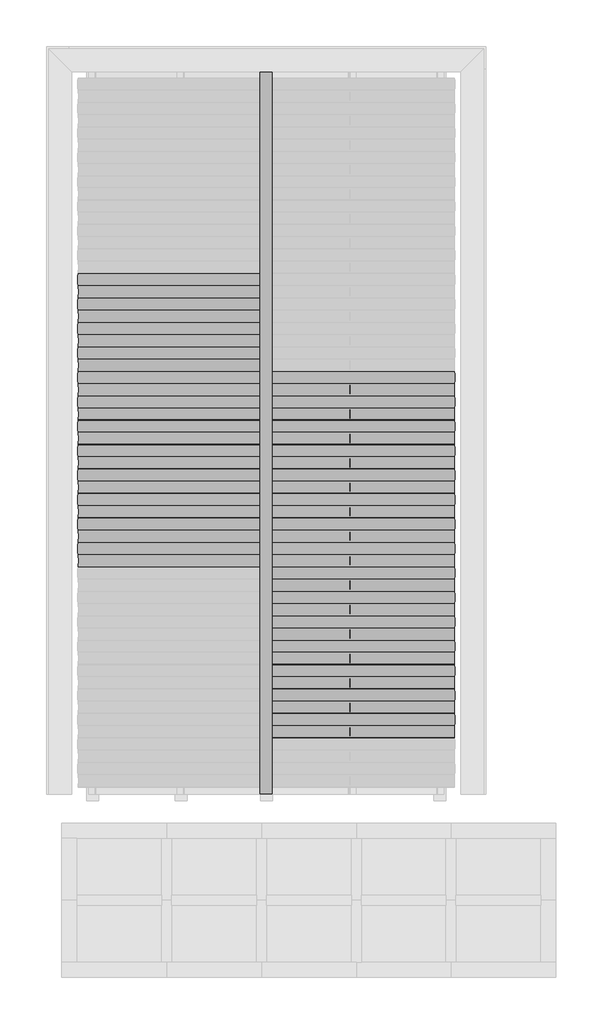
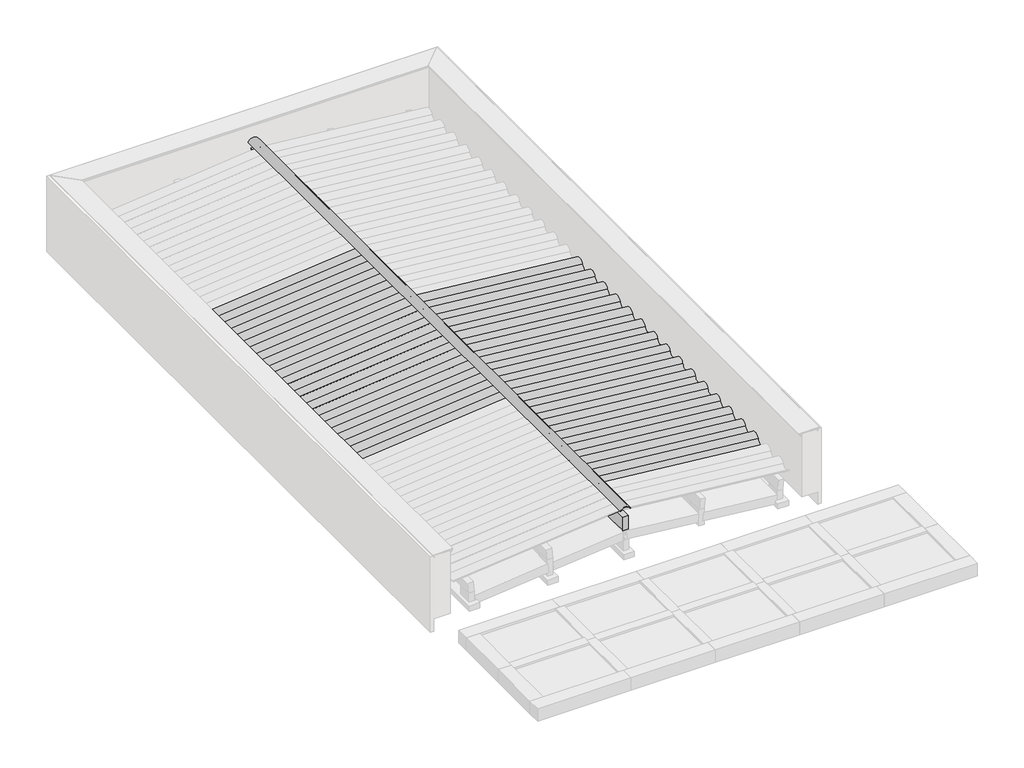
# One storey, part 2 of 3: 34 beams, 6 columns.
"""IFC4 building model written with IfcOpenShell, lengths in millimetres."""

import ifcopenshell
import ifcopenshell.guid

model = None  # the IFC model being written
_history = None  # IfcOwnerHistory: only IFC2X3 demands one
_inside = {}  # id of a spatial element -> (the spatial element, [elements in it])
_under = {}  # id of a project, library or spatial element -> (it, [spatial elements below it])
_declared = {}  # id of a project -> (the project, [libraries it declares])
_typed = {}  # id of a type object -> (the type object, [elements of that type])
_made_of = {}  # id of a material, layer set ... -> (it, [elements and type objects made of it])


def new_model(schema):
    """Start an empty IFC model of exactly this schema.

    Asked for "IFC4X3", IfcOpenShell would pick the latest addendum, in which some entities
    have other attributes; the version numbers below select the first issue.
    IFC2X3 requires an IfcOwnerHistory on every rooted entity: one is made here for all.
    """
    global model, _history
    if schema == "IFC4X3":
        model = ifcopenshell.file(schema_version=(4, 3, 0, 0))
    else:
        model = ifcopenshell.file(schema=schema)
    _inside.clear()
    _under.clear()
    _declared.clear()
    _typed.clear()
    _made_of.clear()
    _history = None
    if model.schema == "IFC2X3":
        org = make("IfcOrganization", Name="unknown")
        user = make(
            "IfcPersonAndOrganization",
            ThePerson=make("IfcPerson", FamilyName="unknown"),
            TheOrganization=org,
        )
        app = make(
            "IfcApplication",
            ApplicationDeveloper=org,
            Version="unknown",
            ApplicationFullName="unknown",
            ApplicationIdentifier="unknown",
        )
        _history = make(
            "IfcOwnerHistory",
            OwningUser=user,
            OwningApplication=app,
            ChangeAction="ADDED",
            CreationDate=0,
        )
    return model


def make(cls, **values):
    """One entity of the class cls with the attributes given. An attribute that is None is left unset."""
    return model.create_entity(
        cls, **{name: value for name, value in values.items() if value is not None}
    )


def rooted(cls, **values):
    """An entity with a GlobalId (a new one), such as an element, a storey or a relation."""
    return make(cls, GlobalId=ifcopenshell.guid.new(), OwnerHistory=_history, **values)


def si_unit(unit_type, name, prefix=None):
    """IfcSIUnit, for example si_unit("LENGTHUNIT", "METRE", prefix="MILLI")."""
    return make("IfcSIUnit", UnitType=unit_type, Prefix=prefix, Name=name)


def assignment(units):
    """IfcUnitAssignment: the units of a project."""
    return None if units is None else make("IfcUnitAssignment", Units=units)


def point(xyz):
    """IfcCartesianPoint."""
    return None if xyz is None else make("IfcCartesianPoint", Coordinates=xyz)


def direction(xyz):
    """IfcDirection."""
    return None if xyz is None else make("IfcDirection", DirectionRatios=xyz)


def frame(location, z_axis=None, x_axis=None):
    """IfcAxis2Placement3D, a coordinate frame: its origin and axes. An axis left out is left unset."""
    return make(
        "IfcAxis2Placement3D",
        Location=point(location),
        Axis=direction(z_axis),
        RefDirection=direction(x_axis),
    )


def frame_2d(location, x_axis=None):
    """IfcAxis2Placement2D, a coordinate frame in the plane: its origin and x axis."""
    return make(
        "IfcAxis2Placement2D", Location=point(location), RefDirection=direction(x_axis)
    )


def origin():
    """The frame at (0, 0, 0) with its axes left unset."""
    return frame((0.0, 0.0, 0.0))


def place(relative_to, where):
    """IfcLocalPlacement: puts the frame where relative to a parent placement (None: the world)."""
    return make(
        "IfcLocalPlacement", PlacementRelTo=relative_to, RelativePlacement=where
    )


def context(
    kind, dimensions, precision=None, world=None, true_north=None, identifier=None
):
    """IfcGeometricRepresentationContext, for example the 3D "Model" context."""
    return make(
        "IfcGeometricRepresentationContext",
        ContextIdentifier=identifier,
        ContextType=kind,
        CoordinateSpaceDimension=dimensions,
        Precision=precision,
        WorldCoordinateSystem=world,
        TrueNorth=true_north,
    )


def project(units=None, contexts=None):
    """IfcProject with its units and contexts."""
    return rooted(
        "IfcProject",
        Name="project",
        RepresentationContexts=contexts,
        UnitsInContext=assignment(units),
    )


def spatial(cls, under=None, at=None, **own):
    """A site, building, storey or space (cls), placed at a placement, below another one or the project."""
    s = rooted(cls, ObjectPlacement=at, **own)
    if under is not None:
        _under.setdefault(under.id(), (under, []))[1].append(s)
    return s


def polyline(points):
    """IfcPolyline through the points."""
    return make("IfcPolyline", Points=[point(p) for p in points])


def circle_curve(where, radius):
    """IfcCircle in the frame where."""
    return make("IfcCircle", Position=where, Radius=radius)


def trimmed(basis, trim1, trim2, sense, master):
    """IfcTrimmedCurve: the piece of a basis curve between two trims."""
    return make(
        "IfcTrimmedCurve",
        BasisCurve=basis,
        Trim1=trim1,
        Trim2=trim2,
        SenseAgreement=sense,
        MasterRepresentation=master,
    )


def segment(curve, same_sense, transition):
    """IfcCompositeCurveSegment."""
    return make(
        "IfcCompositeCurveSegment",
        Transition=transition,
        SameSense=same_sense,
        ParentCurve=curve,
    )


def composite_curve(segments, self_intersect=None):
    """IfcCompositeCurve: segments joined end to end."""
    return make("IfcCompositeCurve", Segments=segments, SelfIntersect=self_intersect)


def outline(outer, holes=None, kind="AREA"):
    """IfcArbitraryClosedProfileDef: a profile drawn as a closed curve; with holes, ...WithVoids."""
    if holes is None:
        return make("IfcArbitraryClosedProfileDef", ProfileType=kind, OuterCurve=outer)
    return make(
        "IfcArbitraryProfileDefWithVoids",
        ProfileType=kind,
        OuterCurve=outer,
        InnerCurves=holes,
    )


def extrude(swept, where, along, depth):
    """IfcExtrudedAreaSolid: the profile swept, set in the frame where, extruded along a direction by depth."""
    return make(
        "IfcExtrudedAreaSolid",
        SweptArea=swept,
        Position=where,
        ExtrudedDirection=direction(along),
        Depth=depth,
    )


def shape(context_of_items, identifier, shape_type, items):
    """IfcShapeRepresentation: the items that make up one representation, for example the "Body"."""
    return make(
        "IfcShapeRepresentation",
        ContextOfItems=context_of_items,
        RepresentationIdentifier=identifier,
        RepresentationType=shape_type,
        Items=items,
    )


def source(mapping_origin, context_of_items, identifier, shape_type, items):
    """IfcRepresentationMap: a shape defined once, which mapped items show again and again."""
    return make(
        "IfcRepresentationMap",
        MappingOrigin=mapping_origin,
        MappedRepresentation=shape(context_of_items, identifier, shape_type, items),
    )


def transform(
    local_origin,
    x_axis=None,
    y_axis=None,
    z_axis=None,
    scale=None,
    scale2=None,
    scale3=None,
    uniform=True,
):
    """IfcCartesianTransformationOperator3D, or its non-uniform kind. x_axis, y_axis, z_axis: its Axis1, 2, 3."""
    if uniform:
        return make(
            "IfcCartesianTransformationOperator3D",
            Axis1=direction(x_axis),
            Axis2=direction(y_axis),
            LocalOrigin=point(local_origin),
            Scale=scale,
            Axis3=direction(z_axis),
        )
    return make(
        "IfcCartesianTransformationOperator3DnonUniform",
        Axis1=direction(x_axis),
        Axis2=direction(y_axis),
        LocalOrigin=point(local_origin),
        Scale=scale,
        Axis3=direction(z_axis),
        Scale2=scale2,
        Scale3=scale3,
    )


def mapped(mapping_source, mapping_target):
    """IfcMappedItem: shows the shape of a source again, moved by a transform."""
    return make(
        "IfcMappedItem", MappingSource=mapping_source, MappingTarget=mapping_target
    )


def made_of(thing, what):
    """Note that an element or type object is made of a material, layer set ...; save() writes the relation."""
    if what is not None:
        _made_of.setdefault(what.id(), (what, []))[1].append(thing)
    return thing


def element(
    cls,
    number,
    at=None,
    inside=None,
    cuts=None,
    type_object=None,
    material=None,
    context=None,
    identifier="Body",
    shape_type=None,
    held_by="IfcProductDefinitionShape",
    body=None,
    shapes=None,
    **own,
):
    """One element of the class cls, such as IfcWall. Its Tag is "e" and its number.

    at: its placement. inside: the storey or other place that contains it. cuts: it is an
    opening in that element (IfcRelVoidsElement). A single representation is given by context,
    identifier, shape_type and body (its items); several are given by shapes. held_by: the class
    of the entity that holds the representations. save() writes the other relations.
    """
    e = rooted(cls, Tag="e%d" % number, ObjectPlacement=at, **own)
    if body is not None:
        shapes = [shape(context, identifier, shape_type, body)]
    if shapes is not None:
        e.Representation = make(held_by, Representations=shapes)
    if inside is not None:
        _inside.setdefault(inside.id(), (inside, []))[1].append(e)
    if cuts is not None:
        rooted(
            "IfcRelVoidsElement", RelatingBuildingElement=cuts, RelatedOpeningElement=e
        )
    if type_object is not None:
        _typed.setdefault(type_object.id(), (type_object, []))[1].append(e)
    return made_of(e, material)


def aggregate(whole, parts):
    """IfcRelAggregates: a whole, such as a stair, and the parts it consists of."""
    return rooted("IfcRelAggregates", RelatingObject=whole, RelatedObjects=parts)


def save(model, path):
    """Write the relations noted so far, then the file.

    IfcRelAggregates (storeys below a building ...), IfcRelContainedInSpatialStructure (elements
    in a storey), IfcRelDefinesByType, IfcRelAssociatesMaterial and IfcRelDeclares: one each for
    every whole, place, type object, material and project.
    """
    for whole, parts in _under.values():
        aggregate(whole, parts)
    for where, things in _inside.values():
        rooted(
            "IfcRelContainedInSpatialStructure",
            RelatedElements=things,
            RelatingStructure=where,
        )
    for kind, things in _typed.values():
        rooted("IfcRelDefinesByType", RelatedObjects=things, RelatingType=kind)
    for what, things in _made_of.values():
        rooted("IfcRelAssociatesMaterial", RelatedObjects=things, RelatingMaterial=what)
    for by, libraries in _declared.values():
        rooted("IfcRelDeclares", RelatingContext=by, RelatedDefinitions=libraries)
    model.write(path)


def cumeeira_telha_ondulada_fibrocimento_28917381(model_context):
    return source(origin(), model_context, "Body", "SweptSolid", [
        extrude(outline(composite_curve([segment(polyline([(58.3970135, 42.4437972), (53.9055884, 40.2467307)]), True, "CONTINUOUS"), segment(trimmed(circle_curve(frame_2d((-1.6029865, 13.0936483)), 61.7939461), [point((53.9055884, 40.2467307))], [point((-57.1115615, 40.2467307))], True, "CARTESIAN"), True, "CONTINUOUS"), segment(polyline([(-57.1115615, 40.2467307), (-61.6029865, 42.4437972)]), True, "CONTINUOUS"), segment(trimmed(circle_curve(frame_2d((-1.6029865, 13.0936483)), 66.7939461), [point((-61.6029865, 42.4437972))], [point((58.3970135, 42.4437972))], False, "CARTESIAN"), True, "CONTINUOUS")], self_intersect=False)), frame((-3626.5, 0.0, 0.0), z_axis=(1.0, 0.0, 0.0), x_axis=(0.0, 1.0, 0.0)), (0.0, 0.0, 1.0), 7253.0),
    ])


def viga_cumeeira_6x16cm_d80f05ee(model_context):
    return source(origin(), model_context, "Body", "SweptSolid", [
        extrude(outline(polyline([(3626.5, 30.0), (3626.5, -30.0), (-3626.5, -30.0), (-3626.5, 30.0), (3626.5, 30.0)])), frame((0.0, 0.0, -80.0), z_axis=(0.0, 0.0, 1.0), x_axis=(1.0, 0.0, 0.0)), (0.0, 0.0, 1.0), 160.0),
    ])


def column_1cffec27(model_context):
    return source(origin(), model_context, "Body", "SweptSolid", [
        extrude(outline(polyline([(30.0, 80.0), (30.0, -80.0), (-30.0, -80.0), (-30.0, 80.0), (30.0, 80.0)])), frame((0.0, 0.0, 3110.0), z_axis=(0.0, 0.0, 1.0), x_axis=(1.0, 0.0, 0.0)), (0.0, 0.0, 1.0), 238.0),
    ])


def column_35730ad5(model_context):
    return source(origin(), model_context, "Body", "SweptSolid", [
        extrude(outline(polyline([(30.0, 80.0), (30.0, -80.0), (-30.0, -80.0), (-30.0, 80.0), (30.0, 80.0)])), frame((0.0, 0.0, 3110.0), z_axis=(0.0, 0.0, 1.0), x_axis=(1.0, 0.0, 0.0)), (0.0, 0.0, 1.0), 197.9),
    ])


def column_00c463e4(model_context):
    return source(origin(), model_context, "Body", "SweptSolid", [
        extrude(outline(polyline([(30.0, 80.0), (30.0, -80.0), (-30.0, -80.0), (-30.0, 80.0), (30.0, 80.0)])), frame((0.0, 0.0, 3110.0), z_axis=(0.0, 0.0, 1.0), x_axis=(1.0, 0.0, 0.0)), (0.0, 0.0, 1.0), 109.8),
    ])


model = new_model("IFC4")

# Units and contexts
model_context = context("Model", 3, world=origin())
ifc_project = project(units=[si_unit("LENGTHUNIT", "METRE", prefix="MILLI")], contexts=[model_context])

# Site, building, storey
site = spatial("IfcSite", under=ifc_project)
building = spatial("IfcBuilding", under=site)
storey = spatial("IfcBuildingStorey", under=building, Name="COB. GARAGEM", Elevation=3050.0)

# Beams
placement = place(None, origin())
element("IfcBeam", 1, ObjectType="Madeira de lei : Berço 6x12cm", at=placement, inside=storey, context=model_context, shape_type="SweptSolid", body=[
    extrude(outline(polyline([(-9620.281307, 4423.9300153), (-9500.281307, 4423.9300153), (-9500.281307, 2423.9300153), (-9620.281307, 2423.9300153), (-9620.281307, 4423.9300153)])), frame((0.0, 0.0, 3050.0), z_axis=(0.0, 0.0, 1.0), x_axis=(1.0, 0.0, 0.0)), (0.0, 0.0, 1.0), 60.0),
])
element("IfcBeam", 2, ObjectType="Madeira de lei : Berço 6x12cm", at=placement, inside=storey, context=model_context, shape_type="SweptSolid", body=[
    extrude(outline(polyline([(-9620.281307, 2423.9300153), (-9500.281307, 2423.9300153), (-9500.281307, 423.9300153), (-9620.281307, 423.9300153), (-9620.281307, 2423.9300153)])), frame((0.0, 0.0, 3050.0), z_axis=(0.0, 0.0, 1.0), x_axis=(1.0, 0.0, 0.0)), (0.0, 0.0, 1.0), 60.0),
])
element("IfcBeam", 3, ObjectType="Madeira de lei : Berço 6x12cm", at=placement, inside=storey, context=model_context, shape_type="SweptSolid", body=[
    extrude(outline(polyline([(-8767.0824227, 4423.9300153), (-8647.0824227, 4423.9300153), (-8647.0824227, 2423.9300153), (-8767.0824227, 2423.9300153), (-8767.0824227, 4423.9300153)])), frame((0.0, 0.0, 3050.0), z_axis=(0.0, 0.0, 1.0), x_axis=(1.0, 0.0, 0.0)), (0.0, 0.0, 1.0), 60.0),
])
element("IfcBeam", 4, ObjectType="Madeira de lei : Berço 6x12cm", at=placement, inside=storey, context=model_context, shape_type="SweptSolid", body=[
    extrude(outline(polyline([(-10473.4801913, 4423.9300153), (-10353.4801913, 4423.9300153), (-10353.4801913, 2423.9300153), (-10473.4801913, 2423.9300153), (-10473.4801913, 4423.9300153)])), frame((0.0, 0.0, 3050.0), z_axis=(0.0, 0.0, 1.0), x_axis=(1.0, 0.0, 0.0)), (0.0, 0.0, 1.0), 60.0),
])
element("IfcBeam", 5, ObjectType="Madeira de lei : Berço 6x12cm", at=placement, inside=storey, context=model_context, shape_type="SweptSolid", body=[
    extrude(outline(polyline([(-11356.5301913, 4423.9300153), (-11236.5301913, 4423.9300153), (-11236.5301913, 2423.9300153), (-11356.5301913, 2423.9300153), (-11356.5301913, 4423.9300153)])), frame((0.0, 0.0, 3050.0), z_axis=(0.0, 0.0, 1.0), x_axis=(1.0, 0.0, 0.0)), (0.0, 0.0, 1.0), 60.0),
])
cumeeira_telha_ondulada_fibrocimento_shape = cumeeira_telha_ondulada_fibrocimento_28917381(model_context)
element("IfcBeam", 6, ObjectType="Cumeeira Telha Ondulada : Fibrocimento", at=placement, inside=storey, context=model_context, shape_type="MappedRepresentation", body=[
    mapped(cumeeira_telha_ondulada_fibrocimento_shape, transform((-9560.281307, 3455.9300153, 3545.9751229), x_axis=(0.0, -1.0, 0.0), y_axis=(1.0, 0.0, 0.0), z_axis=(0.0, 0.0, 1.0))),
])
element("IfcBeam", 7, ObjectType="Telha Ondulada : Fibrocimento", at=placement, inside=storey, context=model_context, shape_type="SweptSolid", body=[
    extrude(outline(composite_curve([segment(trimmed(circle_curve(frame_2d((-58.7002979, -53.2060538)), 66.7939461), [point((-29.350149, 6.7939462))], [point((-29.350149, -113.2060538))], False, "CARTESIAN"), True, "CONTINUOUS"), segment(polyline([(-29.350149, -113.2060538), (-31.5472155, -108.7146288)]), True, "CONTINUOUS"), segment(trimmed(circle_curve(frame_2d((-58.7002979, -53.2060538)), 61.7939461), [point((-31.5472155, -108.7146288))], [point((-31.5472155, 2.3025211))], True, "CARTESIAN"), True, "CONTINUOUS"), segment(trimmed(circle_curve(frame_2d((0.0, 66.7939462)), 71.7939461), [point((-31.5472155, 2.3025211))], [point((-31.5472155, 131.2853712))], False, "CARTESIAN"), True, "CONTINUOUS"), segment(polyline([(-31.5472155, 131.2853712), (-29.350149, 126.7939462)]), True, "CONTINUOUS"), segment(trimmed(circle_curve(frame_2d((0.0, 66.7939462)), 66.7939461), [point((-29.350149, 126.7939462))], [point((-29.350149, 6.7939462))], True, "CARTESIAN"), True, "CONTINUOUS")], self_intersect=False)), frame((-11446.918865, 2229.326948, 3394.3067746), z_axis=(0.9950371902099892, 0.0, 0.09950371902099919), x_axis=(-0.09950371902099919, 0.0, 0.9950371902099892)), (0.0, 0.0, 1.0), 1886.8678854),
])
element("IfcBeam", 8, ObjectType="Telha Ondulada : Fibrocimento", at=placement, inside=storey, context=model_context, shape_type="SweptSolid", body=[
    extrude(outline(composite_curve([segment(trimmed(circle_curve(frame_2d((-58.7002979, -53.2060538)), 66.7939461), [point((-29.350149, 6.7939462))], [point((-29.350149, -113.2060538))], False, "CARTESIAN"), True, "CONTINUOUS"), segment(polyline([(-29.350149, -113.2060538), (-31.5472155, -108.7146288)]), True, "CONTINUOUS"), segment(trimmed(circle_curve(frame_2d((-58.7002979, -53.2060538)), 61.7939461), [point((-31.5472155, -108.7146288))], [point((-31.5472155, 2.3025211))], True, "CARTESIAN"), True, "CONTINUOUS"), segment(trimmed(circle_curve(frame_2d((0.0, 66.7939462)), 71.7939461), [point((-31.5472155, 2.3025211))], [point((-31.5472155, 131.2853712))], False, "CARTESIAN"), True, "CONTINUOUS"), segment(polyline([(-31.5472155, 131.2853712), (-29.350149, 126.7939462)]), True, "CONTINUOUS"), segment(trimmed(circle_curve(frame_2d((0.0, 66.7939462)), 66.7939461), [point((-29.350149, 126.7939462))], [point((-29.350149, 6.7939462))], True, "CARTESIAN"), True, "CONTINUOUS")], self_intersect=False)), frame((-11446.918865, 2473.826948, 3394.3067746), z_axis=(0.9950371902099892, 0.0, 0.09950371902099932), x_axis=(-0.09950371902099932, 0.0, 0.9950371902099892)), (0.0, 0.0, 1.0), 1886.8678854),
])
element("IfcBeam", 9, ObjectType="Telha Ondulada : Fibrocimento", at=placement, inside=storey, context=model_context, shape_type="SweptSolid", body=[
    extrude(outline(composite_curve([segment(trimmed(circle_curve(frame_2d((-58.7002979, -53.2060538)), 66.7939461), [point((-29.350149, 6.7939462))], [point((-29.350149, -113.2060538))], False, "CARTESIAN"), True, "CONTINUOUS"), segment(polyline([(-29.350149, -113.2060538), (-31.5472155, -108.7146288)]), True, "CONTINUOUS"), segment(trimmed(circle_curve(frame_2d((-58.7002979, -53.2060538)), 61.7939461), [point((-31.5472155, -108.7146288))], [point((-31.5472155, 2.3025211))], True, "CARTESIAN"), True, "CONTINUOUS"), segment(trimmed(circle_curve(frame_2d((0.0, 66.7939462)), 71.7939461), [point((-31.5472155, 2.3025211))], [point((-31.5472155, 131.2853712))], False, "CARTESIAN"), True, "CONTINUOUS"), segment(polyline([(-31.5472155, 131.2853712), (-29.350149, 126.7939462)]), True, "CONTINUOUS"), segment(trimmed(circle_curve(frame_2d((0.0, 66.7939462)), 66.7939461), [point((-29.350149, 126.7939462))], [point((-29.350149, 6.7939462))], True, "CARTESIAN"), True, "CONTINUOUS")], self_intersect=False)), frame((-11446.918865, 2718.326948, 3394.3067746), z_axis=(0.9950371902099892, 0.0, 0.09950371902099937), x_axis=(-0.09950371902099937, 0.0, 0.9950371902099892)), (0.0, 0.0, 1.0), 1886.8678854),
])
element("IfcBeam", 10, ObjectType="Telha Ondulada : Fibrocimento", at=placement, inside=storey, context=model_context, shape_type="SweptSolid", body=[
    extrude(outline(composite_curve([segment(trimmed(circle_curve(frame_2d((-58.7002979, -53.2060538)), 66.7939461), [point((-29.350149, 6.7939462))], [point((-29.350149, -113.2060538))], False, "CARTESIAN"), True, "CONTINUOUS"), segment(polyline([(-29.350149, -113.2060538), (-31.5472155, -108.7146288)]), True, "CONTINUOUS"), segment(trimmed(circle_curve(frame_2d((-58.7002979, -53.2060538)), 61.7939461), [point((-31.5472155, -108.7146288))], [point((-31.5472155, 2.3025211))], True, "CARTESIAN"), True, "CONTINUOUS"), segment(trimmed(circle_curve(frame_2d((0.0, 66.7939462)), 71.7939461), [point((-31.5472155, 2.3025211))], [point((-31.5472155, 131.2853712))], False, "CARTESIAN"), True, "CONTINUOUS"), segment(polyline([(-31.5472155, 131.2853712), (-29.350149, 126.7939462)]), True, "CONTINUOUS"), segment(trimmed(circle_curve(frame_2d((0.0, 66.7939462)), 66.7939461), [point((-29.350149, 126.7939462))], [point((-29.350149, 6.7939462))], True, "CARTESIAN"), True, "CONTINUOUS")], self_intersect=False)), frame((-11446.918865, 2962.826948, 3394.3067746), z_axis=(0.9950371902099892, 0.0, 0.09950371902099943), x_axis=(-0.09950371902099943, 0.0, 0.9950371902099892)), (0.0, 0.0, 1.0), 1886.8678854),
])
element("IfcBeam", 11, ObjectType="Telha Ondulada : Fibrocimento", at=placement, inside=storey, context=model_context, shape_type="SweptSolid", body=[
    extrude(outline(composite_curve([segment(trimmed(circle_curve(frame_2d((-58.7002979, -53.2060538)), 66.7939461), [point((-29.350149, 6.7939462))], [point((-29.350149, -113.2060538))], False, "CARTESIAN"), True, "CONTINUOUS"), segment(polyline([(-29.350149, -113.2060538), (-31.5472155, -108.7146288)]), True, "CONTINUOUS"), segment(trimmed(circle_curve(frame_2d((-58.7002979, -53.2060538)), 61.7939461), [point((-31.5472155, -108.7146288))], [point((-31.5472155, 2.3025211))], True, "CARTESIAN"), True, "CONTINUOUS"), segment(trimmed(circle_curve(frame_2d((0.0, 66.7939462)), 71.7939461), [point((-31.5472155, 2.3025211))], [point((-31.5472155, 131.2853712))], False, "CARTESIAN"), True, "CONTINUOUS"), segment(polyline([(-31.5472155, 131.2853712), (-29.350149, 126.7939462)]), True, "CONTINUOUS"), segment(trimmed(circle_curve(frame_2d((0.0, 66.7939462)), 66.7939461), [point((-29.350149, 126.7939462))], [point((-29.350149, 6.7939462))], True, "CARTESIAN"), True, "CONTINUOUS")], self_intersect=False)), frame((-11446.918865, 3207.326948, 3394.3067746), z_axis=(0.9950371902099892, 0.0, 0.09950371902099954), x_axis=(-0.09950371902099954, 0.0, 0.9950371902099892)), (0.0, 0.0, 1.0), 1886.8678854),
])
element("IfcBeam", 12, ObjectType="Telha Ondulada : Fibrocimento", at=placement, inside=storey, context=model_context, shape_type="SweptSolid", body=[
    extrude(outline(composite_curve([segment(trimmed(circle_curve(frame_2d((-58.7002979, -53.2060538)), 66.7939461), [point((-29.350149, 6.7939462))], [point((-29.350149, -113.2060538))], False, "CARTESIAN"), True, "CONTINUOUS"), segment(polyline([(-29.350149, -113.2060538), (-31.5472155, -108.7146288)]), True, "CONTINUOUS"), segment(trimmed(circle_curve(frame_2d((-58.7002979, -53.2060538)), 61.7939461), [point((-31.5472155, -108.7146288))], [point((-31.5472155, 2.3025211))], True, "CARTESIAN"), True, "CONTINUOUS"), segment(trimmed(circle_curve(frame_2d((0.0, 66.7939462)), 71.7939461), [point((-31.5472155, 2.3025211))], [point((-31.5472155, 131.2853712))], False, "CARTESIAN"), True, "CONTINUOUS"), segment(polyline([(-31.5472155, 131.2853712), (-29.350149, 126.7939462)]), True, "CONTINUOUS"), segment(trimmed(circle_curve(frame_2d((0.0, 66.7939462)), 66.7939461), [point((-29.350149, 126.7939462))], [point((-29.350149, 6.7939462))], True, "CARTESIAN"), True, "CONTINUOUS")], self_intersect=False)), frame((-11446.918865, 3451.826948, 3394.3067746), z_axis=(0.9950371902099892, 0.0, 0.09950371902099937), x_axis=(-0.09950371902099937, 0.0, 0.9950371902099892)), (0.0, 0.0, 1.0), 1886.8678854),
])
element("IfcBeam", 13, ObjectType="Telha Ondulada : Fibrocimento", at=placement, inside=storey, context=model_context, shape_type="SweptSolid", body=[
    extrude(outline(composite_curve([segment(trimmed(circle_curve(frame_2d((-58.7002979, -53.2060538)), 66.7939461), [point((-29.350149, 6.7939462))], [point((-29.350149, -113.2060538))], False, "CARTESIAN"), True, "CONTINUOUS"), segment(polyline([(-29.350149, -113.2060538), (-31.5472155, -108.7146288)]), True, "CONTINUOUS"), segment(trimmed(circle_curve(frame_2d((-58.7002979, -53.2060538)), 61.7939461), [point((-31.5472155, -108.7146288))], [point((-31.5472155, 2.3025211))], True, "CARTESIAN"), True, "CONTINUOUS"), segment(trimmed(circle_curve(frame_2d((0.0, 66.7939462)), 71.7939461), [point((-31.5472155, 2.3025211))], [point((-31.5472155, 131.2853712))], False, "CARTESIAN"), True, "CONTINUOUS"), segment(polyline([(-31.5472155, 131.2853712), (-29.350149, 126.7939462)]), True, "CONTINUOUS"), segment(trimmed(circle_curve(frame_2d((0.0, 66.7939462)), 66.7939461), [point((-29.350149, 126.7939462))], [point((-29.350149, 6.7939462))], True, "CARTESIAN"), True, "CONTINUOUS")], self_intersect=False)), frame((-11446.918865, 3696.326948, 3394.3067746), z_axis=(0.9950371902099892, 0.0, 0.09950371902099914), x_axis=(-0.09950371902099914, 0.0, 0.9950371902099892)), (0.0, 0.0, 1.0), 1886.8678854),
])
element("IfcBeam", 14, ObjectType="Telha Ondulada : Fibrocimento", at=placement, inside=storey, context=model_context, shape_type="SweptSolid", body=[
    extrude(outline(composite_curve([segment(trimmed(circle_curve(frame_2d((-58.7002979, -53.2060538)), 66.7939461), [point((-29.350149, 6.7939462))], [point((-29.350149, -113.2060538))], False, "CARTESIAN"), True, "CONTINUOUS"), segment(polyline([(-29.350149, -113.2060538), (-31.5472155, -108.7146288)]), True, "CONTINUOUS"), segment(trimmed(circle_curve(frame_2d((-58.7002979, -53.2060538)), 61.7939461), [point((-31.5472155, -108.7146288))], [point((-31.5472155, 2.3025211))], True, "CARTESIAN"), True, "CONTINUOUS"), segment(trimmed(circle_curve(frame_2d((0.0, 66.7939462)), 71.7939461), [point((-31.5472155, 2.3025211))], [point((-31.5472155, 131.2853712))], False, "CARTESIAN"), True, "CONTINUOUS"), segment(polyline([(-31.5472155, 131.2853712), (-29.350149, 126.7939462)]), True, "CONTINUOUS"), segment(trimmed(circle_curve(frame_2d((0.0, 66.7939462)), 66.7939461), [point((-29.350149, 126.7939462))], [point((-29.350149, 6.7939462))], True, "CARTESIAN"), True, "CONTINUOUS")], self_intersect=False)), frame((-11446.918865, 3940.826948, 3394.3067746), z_axis=(0.9950371902099892, 0.0, 0.09950371902099948), x_axis=(-0.09950371902099948, 0.0, 0.9950371902099892)), (0.0, 0.0, 1.0), 1886.8678854),
])
element("IfcBeam", 15, ObjectType="Telha Ondulada : Fibrocimento", at=placement, inside=storey, context=model_context, shape_type="SweptSolid", body=[
    extrude(outline(composite_curve([segment(trimmed(circle_curve(frame_2d((-58.7002979, -53.2060538)), 66.7939461), [point((-29.350149, 6.7939462))], [point((-29.350149, -113.2060538))], False, "CARTESIAN"), True, "CONTINUOUS"), segment(polyline([(-29.350149, -113.2060538), (-31.5472155, -108.7146288)]), True, "CONTINUOUS"), segment(trimmed(circle_curve(frame_2d((-58.7002979, -53.2060538)), 61.7939461), [point((-31.5472155, -108.7146288))], [point((-31.5472155, 2.3025211))], True, "CARTESIAN"), True, "CONTINUOUS"), segment(trimmed(circle_curve(frame_2d((0.0, 66.7939462)), 71.7939461), [point((-31.5472155, 2.3025211))], [point((-31.5472155, 131.2853712))], False, "CARTESIAN"), True, "CONTINUOUS"), segment(polyline([(-31.5472155, 131.2853712), (-29.350149, 126.7939462)]), True, "CONTINUOUS"), segment(trimmed(circle_curve(frame_2d((0.0, 66.7939462)), 66.7939461), [point((-29.350149, 126.7939462))], [point((-29.350149, 6.7939462))], True, "CARTESIAN"), True, "CONTINUOUS")], self_intersect=False)), frame((-11446.918865, 4185.326948, 3394.3067746), z_axis=(0.9950371902099892, 0.0, 0.09950371902099932), x_axis=(-0.09950371902099932, 0.0, 0.9950371902099892)), (0.0, 0.0, 1.0), 1886.8678854),
])
element("IfcBeam", 16, ObjectType="Telha Ondulada : Fibrocimento", at=placement, inside=storey, context=model_context, shape_type="SweptSolid", body=[
    extrude(outline(composite_curve([segment(trimmed(circle_curve(frame_2d((-58.7002979, -53.2060538)), 66.7939461), [point((-29.350149, 6.7939462))], [point((-29.350149, -113.2060538))], False, "CARTESIAN"), True, "CONTINUOUS"), segment(polyline([(-29.350149, -113.2060538), (-31.5472155, -108.7146288)]), True, "CONTINUOUS"), segment(trimmed(circle_curve(frame_2d((-58.7002979, -53.2060538)), 61.7939461), [point((-31.5472155, -108.7146288))], [point((-31.5472155, 2.3025211))], True, "CARTESIAN"), True, "CONTINUOUS"), segment(trimmed(circle_curve(frame_2d((0.0, 66.7939462)), 71.7939461), [point((-31.5472155, 2.3025211))], [point((-31.5472155, 131.2853712))], False, "CARTESIAN"), True, "CONTINUOUS"), segment(polyline([(-31.5472155, 131.2853712), (-29.350149, 126.7939462)]), True, "CONTINUOUS"), segment(trimmed(circle_curve(frame_2d((0.0, 66.7939462)), 66.7939461), [point((-29.350149, 126.7939462))], [point((-29.350149, 6.7939462))], True, "CARTESIAN"), True, "CONTINUOUS")], self_intersect=False)), frame((-11446.918865, 4429.826948, 3394.3067746), z_axis=(0.9950371902099892, 0.0, 0.09950371902099943), x_axis=(-0.09950371902099943, 0.0, 0.9950371902099892)), (0.0, 0.0, 1.0), 1886.8678854),
])
element("IfcBeam", 17, ObjectType="Telha Ondulada : Fibrocimento", at=placement, inside=storey, context=model_context, shape_type="SweptSolid", body=[
    extrude(outline(composite_curve([segment(trimmed(circle_curve(frame_2d((-58.7002979, -53.2060538)), 66.7939461), [point((-29.350149, 6.7939462))], [point((-29.350149, -113.2060538))], False, "CARTESIAN"), True, "CONTINUOUS"), segment(polyline([(-29.350149, -113.2060538), (-31.5472155, -108.7146288)]), True, "CONTINUOUS"), segment(trimmed(circle_curve(frame_2d((-58.7002979, -53.2060538)), 61.7939461), [point((-31.5472155, -108.7146288))], [point((-31.5472155, 2.3025211))], True, "CARTESIAN"), True, "CONTINUOUS"), segment(trimmed(circle_curve(frame_2d((0.0, 66.7939462)), 71.7939461), [point((-31.5472155, 2.3025211))], [point((-31.5472155, 131.2853712))], False, "CARTESIAN"), True, "CONTINUOUS"), segment(polyline([(-31.5472155, 131.2853712), (-29.350149, 126.7939462)]), True, "CONTINUOUS"), segment(trimmed(circle_curve(frame_2d((0.0, 66.7939462)), 66.7939461), [point((-29.350149, 126.7939462))], [point((-29.350149, 6.7939462))], True, "CARTESIAN"), True, "CONTINUOUS")], self_intersect=False)), frame((-11446.918865, 4674.326948, 3394.3067746), z_axis=(0.9950371902099892, 0.0, 0.09950371902099943), x_axis=(-0.09950371902099943, 0.0, 0.9950371902099892)), (0.0, 0.0, 1.0), 1886.8678854),
])
element("IfcBeam", 18, ObjectType="Telha Ondulada : Fibrocimento", at=placement, inside=storey, context=model_context, shape_type="SweptSolid", body=[
    extrude(outline(composite_curve([segment(trimmed(circle_curve(frame_2d((-58.7002979, -53.2060538)), 66.7939461), [point((-29.350149, 6.7939462))], [point((-29.350149, -113.2060538))], False, "CARTESIAN"), True, "CONTINUOUS"), segment(polyline([(-29.350149, -113.2060538), (-31.5472155, -108.7146288)]), True, "CONTINUOUS"), segment(trimmed(circle_curve(frame_2d((-58.7002979, -53.2060538)), 61.7939461), [point((-31.5472155, -108.7146288))], [point((-31.5472155, 2.3025211))], True, "CARTESIAN"), True, "CONTINUOUS"), segment(trimmed(circle_curve(frame_2d((0.0, 66.7939462)), 71.7939461), [point((-31.5472155, 2.3025211))], [point((-31.5472155, 131.2853712))], False, "CARTESIAN"), True, "CONTINUOUS"), segment(polyline([(-31.5472155, 131.2853712), (-29.350149, 126.7939462)]), True, "CONTINUOUS"), segment(trimmed(circle_curve(frame_2d((0.0, 66.7939462)), 66.7939461), [point((-29.350149, 126.7939462))], [point((-29.350149, 6.7939462))], True, "CARTESIAN"), True, "CONTINUOUS")], self_intersect=False)), frame((-11446.918865, 4918.826948, 3394.3067746), z_axis=(0.9950371902099892, 0.0, 0.09950371902099903), x_axis=(-0.09950371902099903, 0.0, 0.9950371902099892)), (0.0, 0.0, 1.0), 1886.8678854),
])
element("IfcBeam", 19, ObjectType="Telha Ondulada : Fibrocimento", at=placement, inside=storey, context=model_context, shape_type="SweptSolid", body=[
    extrude(outline(composite_curve([segment(trimmed(circle_curve(frame_2d((0.0, 66.7939462)), 66.7939461), [point((29.350149, 6.7939462))], [point((29.350149, 126.7939462))], True, "CARTESIAN"), True, "CONTINUOUS"), segment(polyline([(29.350149, 126.7939462), (31.5472155, 131.2853712)]), True, "CONTINUOUS"), segment(trimmed(circle_curve(frame_2d((0.0, 66.7939462)), 71.7939461), [point((31.5472155, 131.2853712))], [point((31.5472155, 2.3025211))], False, "CARTESIAN"), True, "CONTINUOUS"), segment(trimmed(circle_curve(frame_2d((58.7002979, -53.2060538)), 61.7939461), [point((31.5472155, 2.3025211))], [point((31.5472155, -108.7146288))], True, "CARTESIAN"), True, "CONTINUOUS"), segment(polyline([(31.5472155, -108.7146288), (29.350149, -113.2060538)]), True, "CONTINUOUS"), segment(trimmed(circle_curve(frame_2d((58.7002979, -53.2060538)), 66.7939461), [point((29.350149, -113.2060538))], [point((29.350149, 6.7939462))], False, "CARTESIAN"), True, "CONTINUOUS")], self_intersect=False)), frame((-7673.6437489, 517.826948, 3394.3067746), z_axis=(-0.9950371902099892, 0.0, 0.09950371902099965), x_axis=(-0.09950371902099965, 0.0, -0.9950371902099892)), (0.0, 0.0, 1.0), 1886.8678854),
])
element("IfcBeam", 20, ObjectType="Telha Ondulada : Fibrocimento", at=placement, inside=storey, context=model_context, shape_type="SweptSolid", body=[
    extrude(outline(composite_curve([segment(trimmed(circle_curve(frame_2d((0.0, 66.7939462)), 66.7939461), [point((29.350149, 6.7939462))], [point((29.350149, 126.7939462))], True, "CARTESIAN"), True, "CONTINUOUS"), segment(polyline([(29.350149, 126.7939462), (31.5472155, 131.2853712)]), True, "CONTINUOUS"), segment(trimmed(circle_curve(frame_2d((0.0, 66.7939462)), 71.7939461), [point((31.5472155, 131.2853712))], [point((31.5472155, 2.3025211))], False, "CARTESIAN"), True, "CONTINUOUS"), segment(trimmed(circle_curve(frame_2d((58.7002979, -53.2060538)), 61.7939461), [point((31.5472155, 2.3025211))], [point((31.5472155, -108.7146288))], True, "CARTESIAN"), True, "CONTINUOUS"), segment(polyline([(31.5472155, -108.7146288), (29.350149, -113.2060538)]), True, "CONTINUOUS"), segment(trimmed(circle_curve(frame_2d((58.7002979, -53.2060538)), 66.7939461), [point((29.350149, -113.2060538))], [point((29.350149, 6.7939462))], False, "CARTESIAN"), True, "CONTINUOUS")], self_intersect=False)), frame((-7673.6437489, 762.326948, 3394.3067746), z_axis=(-0.9950371902099892, 0.0, 0.09950371902099965), x_axis=(-0.09950371902099965, 0.0, -0.9950371902099892)), (0.0, 0.0, 1.0), 1886.8678854),
])
element("IfcBeam", 21, ObjectType="Telha Ondulada : Fibrocimento", at=placement, inside=storey, context=model_context, shape_type="SweptSolid", body=[
    extrude(outline(composite_curve([segment(trimmed(circle_curve(frame_2d((0.0, 66.7939462)), 66.7939461), [point((29.350149, 6.7939462))], [point((29.350149, 126.7939462))], True, "CARTESIAN"), True, "CONTINUOUS"), segment(polyline([(29.350149, 126.7939462), (31.5472155, 131.2853712)]), True, "CONTINUOUS"), segment(trimmed(circle_curve(frame_2d((0.0, 66.7939462)), 71.7939461), [point((31.5472155, 131.2853712))], [point((31.5472155, 2.3025211))], False, "CARTESIAN"), True, "CONTINUOUS"), segment(trimmed(circle_curve(frame_2d((58.7002979, -53.2060538)), 61.7939461), [point((31.5472155, 2.3025211))], [point((31.5472155, -108.7146288))], True, "CARTESIAN"), True, "CONTINUOUS"), segment(polyline([(31.5472155, -108.7146288), (29.350149, -113.2060538)]), True, "CONTINUOUS"), segment(trimmed(circle_curve(frame_2d((58.7002979, -53.2060538)), 66.7939461), [point((29.350149, -113.2060538))], [point((29.350149, 6.7939462))], False, "CARTESIAN"), True, "CONTINUOUS")], self_intersect=False)), frame((-7673.6437489, 1006.826948, 3394.3067746), z_axis=(-0.9950371902099892, 0.0, 0.09950371902099965), x_axis=(-0.09950371902099965, 0.0, -0.9950371902099892)), (0.0, 0.0, 1.0), 1886.8678854),
])
element("IfcBeam", 22, ObjectType="Telha Ondulada : Fibrocimento", at=placement, inside=storey, context=model_context, shape_type="SweptSolid", body=[
    extrude(outline(composite_curve([segment(trimmed(circle_curve(frame_2d((0.0, 66.7939462)), 66.7939461), [point((29.350149, 6.7939462))], [point((29.350149, 126.7939462))], True, "CARTESIAN"), True, "CONTINUOUS"), segment(polyline([(29.350149, 126.7939462), (31.5472155, 131.2853712)]), True, "CONTINUOUS"), segment(trimmed(circle_curve(frame_2d((0.0, 66.7939462)), 71.7939461), [point((31.5472155, 131.2853712))], [point((31.5472155, 2.3025211))], False, "CARTESIAN"), True, "CONTINUOUS"), segment(trimmed(circle_curve(frame_2d((58.7002979, -53.2060538)), 61.7939461), [point((31.5472155, 2.3025211))], [point((31.5472155, -108.7146288))], True, "CARTESIAN"), True, "CONTINUOUS"), segment(polyline([(31.5472155, -108.7146288), (29.350149, -113.2060538)]), True, "CONTINUOUS"), segment(trimmed(circle_curve(frame_2d((58.7002979, -53.2060538)), 66.7939461), [point((29.350149, -113.2060538))], [point((29.350149, 6.7939462))], False, "CARTESIAN"), True, "CONTINUOUS")], self_intersect=False)), frame((-7673.6437489, 1251.326948, 3394.3067746), z_axis=(-0.9950371902099892, 0.0, 0.09950371902099965), x_axis=(-0.09950371902099965, 0.0, -0.9950371902099892)), (0.0, 0.0, 1.0), 1886.8678854),
])
element("IfcBeam", 23, ObjectType="Telha Ondulada : Fibrocimento", at=placement, inside=storey, context=model_context, shape_type="SweptSolid", body=[
    extrude(outline(composite_curve([segment(trimmed(circle_curve(frame_2d((0.0, 66.7939462)), 66.7939461), [point((29.350149, 6.7939462))], [point((29.350149, 126.7939462))], True, "CARTESIAN"), True, "CONTINUOUS"), segment(polyline([(29.350149, 126.7939462), (31.5472155, 131.2853712)]), True, "CONTINUOUS"), segment(trimmed(circle_curve(frame_2d((0.0, 66.7939462)), 71.7939461), [point((31.5472155, 131.2853712))], [point((31.5472155, 2.3025211))], False, "CARTESIAN"), True, "CONTINUOUS"), segment(trimmed(circle_curve(frame_2d((58.7002979, -53.2060538)), 61.7939461), [point((31.5472155, 2.3025211))], [point((31.5472155, -108.7146288))], True, "CARTESIAN"), True, "CONTINUOUS"), segment(polyline([(31.5472155, -108.7146288), (29.350149, -113.2060538)]), True, "CONTINUOUS"), segment(trimmed(circle_curve(frame_2d((58.7002979, -53.2060538)), 66.7939461), [point((29.350149, -113.2060538))], [point((29.350149, 6.7939462))], False, "CARTESIAN"), True, "CONTINUOUS")], self_intersect=False)), frame((-7673.6437489, 1495.826948, 3394.3067746), z_axis=(-0.9950371902099892, 0.0, 0.09950371902099965), x_axis=(-0.09950371902099965, 0.0, -0.9950371902099892)), (0.0, 0.0, 1.0), 1886.8678854),
])
element("IfcBeam", 24, ObjectType="Telha Ondulada : Fibrocimento", at=placement, inside=storey, context=model_context, shape_type="SweptSolid", body=[
    extrude(outline(composite_curve([segment(trimmed(circle_curve(frame_2d((0.0, 66.7939462)), 66.7939461), [point((29.350149, 6.7939462))], [point((29.350149, 126.7939462))], True, "CARTESIAN"), True, "CONTINUOUS"), segment(polyline([(29.350149, 126.7939462), (31.5472155, 131.2853712)]), True, "CONTINUOUS"), segment(trimmed(circle_curve(frame_2d((0.0, 66.7939462)), 71.7939461), [point((31.5472155, 131.2853712))], [point((31.5472155, 2.3025211))], False, "CARTESIAN"), True, "CONTINUOUS"), segment(trimmed(circle_curve(frame_2d((58.7002979, -53.2060538)), 61.7939461), [point((31.5472155, 2.3025211))], [point((31.5472155, -108.7146288))], True, "CARTESIAN"), True, "CONTINUOUS"), segment(polyline([(31.5472155, -108.7146288), (29.350149, -113.2060538)]), True, "CONTINUOUS"), segment(trimmed(circle_curve(frame_2d((58.7002979, -53.2060538)), 66.7939461), [point((29.350149, -113.2060538))], [point((29.350149, 6.7939462))], False, "CARTESIAN"), True, "CONTINUOUS")], self_intersect=False)), frame((-7673.6437489, 1740.326948, 3394.3067746), z_axis=(-0.9950371902099892, 0.0, 0.09950371902099965), x_axis=(-0.09950371902099965, 0.0, -0.9950371902099892)), (0.0, 0.0, 1.0), 1886.8678854),
])
element("IfcBeam", 25, ObjectType="Telha Ondulada : Fibrocimento", at=placement, inside=storey, context=model_context, shape_type="SweptSolid", body=[
    extrude(outline(composite_curve([segment(trimmed(circle_curve(frame_2d((0.0, 66.7939462)), 66.7939461), [point((29.350149, 6.7939462))], [point((29.350149, 126.7939462))], True, "CARTESIAN"), True, "CONTINUOUS"), segment(polyline([(29.350149, 126.7939462), (31.5472155, 131.2853712)]), True, "CONTINUOUS"), segment(trimmed(circle_curve(frame_2d((0.0, 66.7939462)), 71.7939461), [point((31.5472155, 131.2853712))], [point((31.5472155, 2.3025211))], False, "CARTESIAN"), True, "CONTINUOUS"), segment(trimmed(circle_curve(frame_2d((58.7002979, -53.2060538)), 61.7939461), [point((31.5472155, 2.3025211))], [point((31.5472155, -108.7146288))], True, "CARTESIAN"), True, "CONTINUOUS"), segment(polyline([(31.5472155, -108.7146288), (29.350149, -113.2060538)]), True, "CONTINUOUS"), segment(trimmed(circle_curve(frame_2d((58.7002979, -53.2060538)), 66.7939461), [point((29.350149, -113.2060538))], [point((29.350149, 6.7939462))], False, "CARTESIAN"), True, "CONTINUOUS")], self_intersect=False)), frame((-7673.6437489, 1984.826948, 3394.3067746), z_axis=(-0.9950371902099892, 0.0, 0.09950371902099965), x_axis=(-0.09950371902099965, 0.0, -0.9950371902099892)), (0.0, 0.0, 1.0), 1886.8678854),
])
element("IfcBeam", 26, ObjectType="Telha Ondulada : Fibrocimento", at=placement, inside=storey, context=model_context, shape_type="SweptSolid", body=[
    extrude(outline(composite_curve([segment(trimmed(circle_curve(frame_2d((0.0, 66.7939462)), 66.7939461), [point((29.350149, 6.7939462))], [point((29.350149, 126.7939462))], True, "CARTESIAN"), True, "CONTINUOUS"), segment(polyline([(29.350149, 126.7939462), (31.5472155, 131.2853712)]), True, "CONTINUOUS"), segment(trimmed(circle_curve(frame_2d((0.0, 66.7939462)), 71.7939461), [point((31.5472155, 131.2853712))], [point((31.5472155, 2.3025211))], False, "CARTESIAN"), True, "CONTINUOUS"), segment(trimmed(circle_curve(frame_2d((58.7002979, -53.2060538)), 61.7939461), [point((31.5472155, 2.3025211))], [point((31.5472155, -108.7146288))], True, "CARTESIAN"), True, "CONTINUOUS"), segment(polyline([(31.5472155, -108.7146288), (29.350149, -113.2060538)]), True, "CONTINUOUS"), segment(trimmed(circle_curve(frame_2d((58.7002979, -53.2060538)), 66.7939461), [point((29.350149, -113.2060538))], [point((29.350149, 6.7939462))], False, "CARTESIAN"), True, "CONTINUOUS")], self_intersect=False)), frame((-7673.6437489, 2229.326948, 3394.3067746), z_axis=(-0.9950371902099892, 0.0, 0.09950371902099965), x_axis=(-0.09950371902099965, 0.0, -0.9950371902099892)), (0.0, 0.0, 1.0), 1886.8678854),
])
element("IfcBeam", 27, ObjectType="Telha Ondulada : Fibrocimento", at=placement, inside=storey, context=model_context, shape_type="SweptSolid", body=[
    extrude(outline(composite_curve([segment(trimmed(circle_curve(frame_2d((0.0, 66.7939462)), 66.7939461), [point((29.350149, 6.7939462))], [point((29.350149, 126.7939462))], True, "CARTESIAN"), True, "CONTINUOUS"), segment(polyline([(29.350149, 126.7939462), (31.5472155, 131.2853712)]), True, "CONTINUOUS"), segment(trimmed(circle_curve(frame_2d((0.0, 66.7939462)), 71.7939461), [point((31.5472155, 131.2853712))], [point((31.5472155, 2.3025211))], False, "CARTESIAN"), True, "CONTINUOUS"), segment(trimmed(circle_curve(frame_2d((58.7002979, -53.2060538)), 61.7939461), [point((31.5472155, 2.3025211))], [point((31.5472155, -108.7146288))], True, "CARTESIAN"), True, "CONTINUOUS"), segment(polyline([(31.5472155, -108.7146288), (29.350149, -113.2060538)]), True, "CONTINUOUS"), segment(trimmed(circle_curve(frame_2d((58.7002979, -53.2060538)), 66.7939461), [point((29.350149, -113.2060538))], [point((29.350149, 6.7939462))], False, "CARTESIAN"), True, "CONTINUOUS")], self_intersect=False)), frame((-7673.6437489, 2473.826948, 3394.3067746), z_axis=(-0.9950371902099892, 0.0, 0.09950371902099965), x_axis=(-0.09950371902099965, 0.0, -0.9950371902099892)), (0.0, 0.0, 1.0), 1886.8678854),
])
element("IfcBeam", 28, ObjectType="Telha Ondulada : Fibrocimento", at=placement, inside=storey, context=model_context, shape_type="SweptSolid", body=[
    extrude(outline(composite_curve([segment(trimmed(circle_curve(frame_2d((0.0, 66.7939462)), 66.7939461), [point((29.350149, 6.7939462))], [point((29.350149, 126.7939462))], True, "CARTESIAN"), True, "CONTINUOUS"), segment(polyline([(29.350149, 126.7939462), (31.5472155, 131.2853712)]), True, "CONTINUOUS"), segment(trimmed(circle_curve(frame_2d((0.0, 66.7939462)), 71.7939461), [point((31.5472155, 131.2853712))], [point((31.5472155, 2.3025211))], False, "CARTESIAN"), True, "CONTINUOUS"), segment(trimmed(circle_curve(frame_2d((58.7002979, -53.2060538)), 61.7939461), [point((31.5472155, 2.3025211))], [point((31.5472155, -108.7146288))], True, "CARTESIAN"), True, "CONTINUOUS"), segment(polyline([(31.5472155, -108.7146288), (29.350149, -113.2060538)]), True, "CONTINUOUS"), segment(trimmed(circle_curve(frame_2d((58.7002979, -53.2060538)), 66.7939461), [point((29.350149, -113.2060538))], [point((29.350149, 6.7939462))], False, "CARTESIAN"), True, "CONTINUOUS")], self_intersect=False)), frame((-7673.6437489, 2718.326948, 3394.3067746), z_axis=(-0.9950371902099892, 0.0, 0.09950371902099965), x_axis=(-0.09950371902099965, 0.0, -0.9950371902099892)), (0.0, 0.0, 1.0), 1886.8678854),
])
element("IfcBeam", 29, ObjectType="Telha Ondulada : Fibrocimento", at=placement, inside=storey, context=model_context, shape_type="SweptSolid", body=[
    extrude(outline(composite_curve([segment(trimmed(circle_curve(frame_2d((0.0, 66.7939462)), 66.7939461), [point((29.350149, 6.7939462))], [point((29.350149, 126.7939462))], True, "CARTESIAN"), True, "CONTINUOUS"), segment(polyline([(29.350149, 126.7939462), (31.5472155, 131.2853712)]), True, "CONTINUOUS"), segment(trimmed(circle_curve(frame_2d((0.0, 66.7939462)), 71.7939461), [point((31.5472155, 131.2853712))], [point((31.5472155, 2.3025211))], False, "CARTESIAN"), True, "CONTINUOUS"), segment(trimmed(circle_curve(frame_2d((58.7002979, -53.2060538)), 61.7939461), [point((31.5472155, 2.3025211))], [point((31.5472155, -108.7146288))], True, "CARTESIAN"), True, "CONTINUOUS"), segment(polyline([(31.5472155, -108.7146288), (29.350149, -113.2060538)]), True, "CONTINUOUS"), segment(trimmed(circle_curve(frame_2d((58.7002979, -53.2060538)), 66.7939461), [point((29.350149, -113.2060538))], [point((29.350149, 6.7939462))], False, "CARTESIAN"), True, "CONTINUOUS")], self_intersect=False)), frame((-7673.6437489, 2962.826948, 3394.3067746), z_axis=(-0.9950371902099892, 0.0, 0.09950371902099965), x_axis=(-0.09950371902099965, 0.0, -0.9950371902099892)), (0.0, 0.0, 1.0), 1886.8678854),
])
element("IfcBeam", 30, ObjectType="Telha Ondulada : Fibrocimento", at=placement, inside=storey, context=model_context, shape_type="SweptSolid", body=[
    extrude(outline(composite_curve([segment(trimmed(circle_curve(frame_2d((0.0, 66.7939462)), 66.7939461), [point((29.350149, 6.7939462))], [point((29.350149, 126.7939462))], True, "CARTESIAN"), True, "CONTINUOUS"), segment(polyline([(29.350149, 126.7939462), (31.5472155, 131.2853712)]), True, "CONTINUOUS"), segment(trimmed(circle_curve(frame_2d((0.0, 66.7939462)), 71.7939461), [point((31.5472155, 131.2853712))], [point((31.5472155, 2.3025211))], False, "CARTESIAN"), True, "CONTINUOUS"), segment(trimmed(circle_curve(frame_2d((58.7002979, -53.2060538)), 61.7939461), [point((31.5472155, 2.3025211))], [point((31.5472155, -108.7146288))], True, "CARTESIAN"), True, "CONTINUOUS"), segment(polyline([(31.5472155, -108.7146288), (29.350149, -113.2060538)]), True, "CONTINUOUS"), segment(trimmed(circle_curve(frame_2d((58.7002979, -53.2060538)), 66.7939461), [point((29.350149, -113.2060538))], [point((29.350149, 6.7939462))], False, "CARTESIAN"), True, "CONTINUOUS")], self_intersect=False)), frame((-7673.6437489, 3207.326948, 3394.3067746), z_axis=(-0.9950371902099892, 0.0, 0.09950371902099965), x_axis=(-0.09950371902099965, 0.0, -0.9950371902099892)), (0.0, 0.0, 1.0), 1886.8678854),
])
element("IfcBeam", 31, ObjectType="Telha Ondulada : Fibrocimento", at=placement, inside=storey, context=model_context, shape_type="SweptSolid", body=[
    extrude(outline(composite_curve([segment(trimmed(circle_curve(frame_2d((0.0, 66.7939462)), 66.7939461), [point((29.350149, 6.7939462))], [point((29.350149, 126.7939462))], True, "CARTESIAN"), True, "CONTINUOUS"), segment(polyline([(29.350149, 126.7939462), (31.5472155, 131.2853712)]), True, "CONTINUOUS"), segment(trimmed(circle_curve(frame_2d((0.0, 66.7939462)), 71.7939461), [point((31.5472155, 131.2853712))], [point((31.5472155, 2.3025211))], False, "CARTESIAN"), True, "CONTINUOUS"), segment(trimmed(circle_curve(frame_2d((58.7002979, -53.2060538)), 61.7939461), [point((31.5472155, 2.3025211))], [point((31.5472155, -108.7146288))], True, "CARTESIAN"), True, "CONTINUOUS"), segment(polyline([(31.5472155, -108.7146288), (29.350149, -113.2060538)]), True, "CONTINUOUS"), segment(trimmed(circle_curve(frame_2d((58.7002979, -53.2060538)), 66.7939461), [point((29.350149, -113.2060538))], [point((29.350149, 6.7939462))], False, "CARTESIAN"), True, "CONTINUOUS")], self_intersect=False)), frame((-7673.6437489, 3451.826948, 3394.3067746), z_axis=(-0.9950371902099892, 0.0, 0.09950371902099965), x_axis=(-0.09950371902099965, 0.0, -0.9950371902099892)), (0.0, 0.0, 1.0), 1886.8678854),
])
element("IfcBeam", 32, ObjectType="Telha Ondulada : Fibrocimento", at=placement, inside=storey, context=model_context, shape_type="SweptSolid", body=[
    extrude(outline(composite_curve([segment(trimmed(circle_curve(frame_2d((0.0, 66.7939462)), 66.7939461), [point((29.350149, 6.7939462))], [point((29.350149, 126.7939462))], True, "CARTESIAN"), True, "CONTINUOUS"), segment(polyline([(29.350149, 126.7939462), (31.5472155, 131.2853712)]), True, "CONTINUOUS"), segment(trimmed(circle_curve(frame_2d((0.0, 66.7939462)), 71.7939461), [point((31.5472155, 131.2853712))], [point((31.5472155, 2.3025211))], False, "CARTESIAN"), True, "CONTINUOUS"), segment(trimmed(circle_curve(frame_2d((58.7002979, -53.2060538)), 61.7939461), [point((31.5472155, 2.3025211))], [point((31.5472155, -108.7146288))], True, "CARTESIAN"), True, "CONTINUOUS"), segment(polyline([(31.5472155, -108.7146288), (29.350149, -113.2060538)]), True, "CONTINUOUS"), segment(trimmed(circle_curve(frame_2d((58.7002979, -53.2060538)), 66.7939461), [point((29.350149, -113.2060538))], [point((29.350149, 6.7939462))], False, "CARTESIAN"), True, "CONTINUOUS")], self_intersect=False)), frame((-7673.6437489, 3696.326948, 3394.3067746), z_axis=(-0.9950371902099892, 0.0, 0.09950371902099965), x_axis=(-0.09950371902099965, 0.0, -0.9950371902099892)), (0.0, 0.0, 1.0), 1886.8678854),
])
element("IfcBeam", 33, ObjectType="Telha Ondulada : Fibrocimento", at=placement, inside=storey, context=model_context, shape_type="SweptSolid", body=[
    extrude(outline(composite_curve([segment(trimmed(circle_curve(frame_2d((0.0, 66.7939462)), 66.7939461), [point((29.350149, 6.7939462))], [point((29.350149, 126.7939462))], True, "CARTESIAN"), True, "CONTINUOUS"), segment(polyline([(29.350149, 126.7939462), (31.5472155, 131.2853712)]), True, "CONTINUOUS"), segment(trimmed(circle_curve(frame_2d((0.0, 66.7939462)), 71.7939461), [point((31.5472155, 131.2853712))], [point((31.5472155, 2.3025211))], False, "CARTESIAN"), True, "CONTINUOUS"), segment(trimmed(circle_curve(frame_2d((58.7002979, -53.2060538)), 61.7939461), [point((31.5472155, 2.3025211))], [point((31.5472155, -108.7146288))], True, "CARTESIAN"), True, "CONTINUOUS"), segment(polyline([(31.5472155, -108.7146288), (29.350149, -113.2060538)]), True, "CONTINUOUS"), segment(trimmed(circle_curve(frame_2d((58.7002979, -53.2060538)), 66.7939461), [point((29.350149, -113.2060538))], [point((29.350149, 6.7939462))], False, "CARTESIAN"), True, "CONTINUOUS")], self_intersect=False)), frame((-7673.6437489, 3940.826948, 3394.3067746), z_axis=(-0.9950371902099892, 0.0, 0.09950371902099965), x_axis=(-0.09950371902099965, 0.0, -0.9950371902099892)), (0.0, 0.0, 1.0), 1886.8678854),
])
viga_cumeeira_6x16cm_shape = viga_cumeeira_6x16cm_d80f05ee(model_context)
element("IfcBeam", 34, ObjectType="Madeira de lei : Viga Cumeeira 6x16cm", at=placement, inside=storey, context=model_context, shape_type="MappedRepresentation", body=[
    mapped(viga_cumeeira_6x16cm_shape, transform((-9560.281307, 3455.9300153, 3427.8), x_axis=(0.0, -1.0, 0.0), y_axis=(1.0, 0.0, 0.0), z_axis=(0.0, 0.0, 1.0))),
])

# Columns
column_shape = column_1cffec27(model_context)
element("IfcColumn", 35, ObjectType="Madeira de lei-Coluna : Pontalete 6X16cm", at=placement, inside=storey, context=model_context, shape_type="MappedRepresentation", body=[
    mapped(column_shape, transform((-9560.281307, 3423.9300153, 0.0), x_axis=(1.0, 0.0, 0.0), y_axis=(0.0, 1.0, 0.0), z_axis=(0.0, 0.0, 1.0))),
])
element("IfcColumn", 36, ObjectType="Madeira de lei-Coluna : Pontalete 6X16cm", at=placement, inside=storey, context=model_context, shape_type="MappedRepresentation", body=[
    mapped(column_shape, transform((-9560.281307, 1423.9300153, 0.0), x_axis=(1.0, 0.0, 0.0), y_axis=(0.0, 1.0, 0.0), z_axis=(0.0, 0.0, 1.0))),
])
column_2_shape = column_35730ad5(model_context)
element("IfcColumn", 37, ObjectType="Madeira de lei-Coluna : Pontalete 6X16cm", at=placement, inside=storey, context=model_context, shape_type="MappedRepresentation", body=[
    mapped(column_2_shape, transform((-8707.0824227, 3423.9300153, 0.0), x_axis=(1.0, 0.0, 0.0), y_axis=(0.0, 1.0, 0.0), z_axis=(0.0, 0.0, 1.0))),
])
element("IfcColumn", 38, ObjectType="Madeira de lei-Coluna : Pontalete 6X16cm", at=placement, inside=storey, context=model_context, shape_type="MappedRepresentation", body=[
    mapped(column_2_shape, transform((-8707.0824227, 1423.9300153, 0.0), x_axis=(1.0, 0.0, 0.0), y_axis=(0.0, 1.0, 0.0), z_axis=(0.0, 0.0, 1.0))),
])
element("IfcColumn", 39, ObjectType="Madeira de lei-Coluna : Pontalete 6X16cm", at=placement, inside=storey, context=model_context, shape_type="MappedRepresentation", body=[
    mapped(column_2_shape, transform((-10413.4801913, 3423.9300153, 0.0), x_axis=(1.0, 0.0, 0.0), y_axis=(0.0, 1.0, 0.0), z_axis=(0.0, 0.0, 1.0))),
])
column_3_shape = column_00c463e4(model_context)
element("IfcColumn", 40, ObjectType="Madeira de lei-Coluna : Pontalete 6X16cm", at=placement, inside=storey, context=model_context, shape_type="MappedRepresentation", body=[
    mapped(column_3_shape, transform((-11296.5301913, 3423.9300153, 0.0), x_axis=(1.0, 0.0, 0.0), y_axis=(0.0, 1.0, 0.0), z_axis=(0.0, 0.0, 1.0))),
])

save(model, "model.ifc")

# Revit data of these elements
# Type "Madeira de lei : Berço 6x12cm"
#   A = 0.02 m²
#   Length [instance default] = 1.524 m
#   b = 0.06 m
#   d = 0.12 m
#   Structural Material [instance default] = none
#   Assembly Code = ""
# Type "Cumeeira Telha Ondulada : Fibrocimento"
#   Cost = 5
#   Length [instance default] = 1.524 m
#   b = 0.07 m
#   h = 0.16 m
#   Structural Material = .TELHA DE FIBROCIMENTO
#   Assembly Code = ""
# Type "Telha Ondulada : Fibrocimento"
#   Description = "TELHA ONDULADA FIBROCIMENTO"
#   Cost = 5
#   Length [instance default] = 1.524 m
#   b = 0.07 m
#   h = 0.16 m
#   Structural Material = .TELHA DE FIBROCIMENTO
#   Assembly Code = ""
# Type "Madeira de lei : Viga Cumeeira 6x16cm"
#   A = 0.02 m²
#   Length [instance default] = 1.524 m
#   b = 0.06 m
#   d = 0.16 m
#   Structural Material [instance default] = none
#   Assembly Code = ""
# Type "Madeira de lei-Coluna : Pontalete 6X16cm"
#   A = 0.01952 m²
#   b = 0.06 m
#   d = 0.16 m
#   Structural Material [instance default] = none
#   Assembly Code = ""
# Elements 1, 2, 3, 4, 5 (IfcBeam, "Madeira de lei : Berço 6x12cm")
#   Comments = ""
#   Uso = "TELHADOS ESTRUTURAS"
#   Compr Cmcl = 6.00 m
#   Structural Material = .MADEIRAMENTO
#   Phase Created = CC_AP
#   Materials on its faces: ".MADEIRAMENTO"
# Element 6 (IfcBeam, "Cumeeira Telha Ondulada : Fibrocimento")
#   Comments = ""
#   Uso = "TELHADOS TELHAS"
#   Phase Created = CC_AP
#   Materials on its faces: ".TELHA DE FIBROCIMENTO"
# Elements 7, 8, 9, 10, 11, 12, 13, 14, 15, 16, 17, 18, 19, 20, 21, 22, 23, 24, 25, 26, 27, 28, 29, 30, 31, 32, 33 (IfcBeam, "Telha Ondulada : Fibrocimento")
#   Uso = "TELHADOS TELHAS"
#   Phase Created = CC_AP
#   Materials on its faces: ".TELHA DE FIBROCIMENTO"
# Element 34 (IfcBeam, "Madeira de lei : Viga Cumeeira 6x16cm")
#   Comments = ""
#   Uso = "TELHADOS MADEIRAMENTO"
#   Compr Cmcl = 7.50 m
#   Structural Material = .MADEIRAMENTO
#   Phase Created = CC_AP
#   Materials on its faces: ".MADEIRAMENTO"
# Elements 35, 36, 37, 38, 39, 40 (IfcColumn, "Madeira de lei-Coluna : Pontalete 6X16cm")
#   Comments = ""
#   Uso = "TELHADOS ESTRUTURAS"
#   Compr Cmcl = 2.00 m
#   Structural Material = .MADEIRAMENTO
#   Phase Created = CC_AP
#   Materials on its faces: ".MADEIRAMENTO"
# Materials
#   ".TELHA DE FIBROCIMENTO": class "CC_TELHADO", colour RGB 77 77 76, transparency 0, Description = "TELHA ONDULADA FIBROCIMENTO", Cost = 0
#   ".MADEIRAMENTO": class ".CC_MADEIRAS", colour RGB 212 179 113, transparency 0, Cost = 0
# Room, not placed, phase "CC_AP", upper offset 0.00 m, lower offset 0.00 m
#   Number = "31"
#   Name = "Room"
# Room, not placed, phase "CC_AP", upper offset 0.00 m, lower offset 0.00 m
#   Number = "34"
#   Name = "Room"
